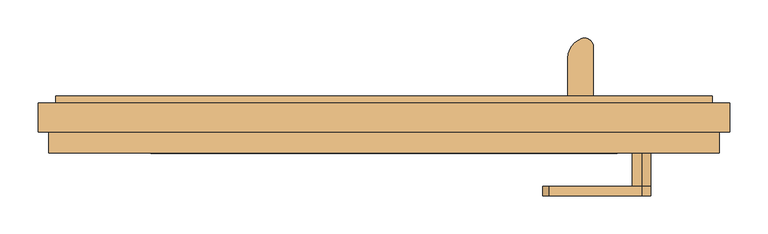
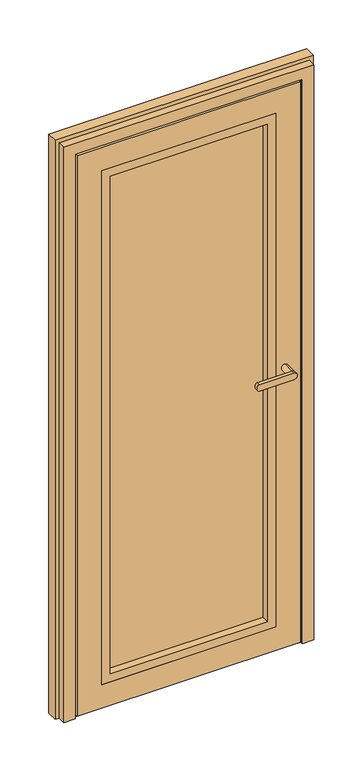
"""IFC4 building model written with IfcOpenShell, lengths in millimetres: door geometry, Schueco_FWS_ADS-75-BL-SimplySmart_inw_Family-01 : FWS SI insert unit."""

from ifc_helpers import new_model, si_unit, point, frame, frame_2d, origin, place, context, project, spatial, polyline, circle_curve, ellipse_curve, trimmed, segment, composite_curve, outline, extrude, faceted_brep, source, transform, mapped, element, save
from ifc_brep_helpers import plane_surface, cylinder_surface, extruded_surface, advanced_brep


def door_fb62e3df(model_context):
    return source(origin(), model_context, "Body", "SolidModel", [
        extrude(outline(composite_curve([segment(polyline([(241.3327032, 8.9997177), (241.3327032, 59.1618682)]), True, "CONTINUOUS"), segment(trimmed(circle_curve(frame_2d((268.5111209, 59.1618682)), 27.1784177), [point((241.3327032, 59.1618682))], [point((258.9740253, 84.6120194))], False, "CARTESIAN"), True, "CONTINUOUS"), segment(trimmed(circle_curve(frame_2d((263.0515262, 73.7310321)), 11.6198924), [point((258.9740253, 84.6120194))], [point((274.6714186, 73.7310321))], False, "CARTESIAN"), True, "CONTINUOUS"), segment(polyline([(274.6714186, 73.7310321), (274.6714186, 8.9997177), (241.3327032, 8.9997177)]), True, "CONTINUOUS")], self_intersect=False)), frame((0.0, 0.0, 2036.9340013), z_axis=(0.0, 0.0, 1.0), x_axis=(1.0, 0.0, 0.0)), (0.0, 0.0, 1.0), 4.0),
        extrude(outline(polyline([(241.3327032, 12.9997177), (274.6714186, 12.9997177), (274.6714186, 8.9997177), (241.3327032, 8.9997177), (241.3327032, 12.9997177)])), frame((0.0, 0.0, 2006.9340013), z_axis=(0.0, 0.0, 1.0), x_axis=(1.0, 0.0, 0.0)), (0.0, 0.0, 1.0), 30.0),
        extrude(outline(polyline([(241.3327032, 12.9997177), (274.6714186, 12.9997177), (274.6714186, 8.9997177), (241.3327032, 8.9997177), (241.3327032, 12.9997177)])), frame((0.0, 0.0, 56.9340013), z_axis=(0.0, 0.0, 1.0), x_axis=(1.0, 0.0, 0.0)), (0.0, 0.0, 1.0), 30.0),
        extrude(outline(composite_curve([segment(polyline([(241.3327032, 8.9997177), (241.3327032, 59.1618682)]), True, "CONTINUOUS"), segment(trimmed(circle_curve(frame_2d((268.5111209, 59.1618682)), 27.1784177), [point((241.3327032, 59.1618682))], [point((258.9740253, 84.6120194))], False, "CARTESIAN"), True, "CONTINUOUS"), segment(trimmed(circle_curve(frame_2d((263.0515262, 73.7310321)), 11.6198924), [point((258.9740253, 84.6120194))], [point((274.6714186, 73.7310321))], False, "CARTESIAN"), True, "CONTINUOUS"), segment(polyline([(274.6714186, 73.7310321), (274.6714186, 8.9997177), (241.3327032, 8.9997177)]), True, "CONTINUOUS")], self_intersect=False)), frame((0.0, 0.0, 52.9340013), z_axis=(0.0, 0.0, 1.0), x_axis=(1.0, 0.0, 0.0)), (0.0, 0.0, 1.0), 4.0),
        advanced_brep(
        [(270.7171028, 57.5977179, 2036.9340013), (245.2829507, 72.2821425, 2036.9340013), (270.7171028, 57.5977179, 56.9340013), (245.2829507, 72.2821425, 56.9340013)],
        [
            (0, 1, ellipse_curve(frame((258.0000268, 64.9399302, 2036.9340013), z_axis=(0.0, 0.0, 1.0000000000000002), x_axis=(0.5000002582658958, 0.866025254674503, 0.0)), 21.5840887, 14.6844171)),
            (1, 0, ellipse_curve(frame((258.0000268, 64.9399302, 2036.9340013), z_axis=(0.0, 0.0, 1.0000000000000002), x_axis=(0.5000002582658958, 0.866025254674503, 0.0)), 21.5840887, 14.6844171)),
            (2, 3, ellipse_curve(frame((258.0000268, 64.9399302, 56.9340013), z_axis=(0.0, 0.0, -1.0000000000000002), x_axis=(-0.866025254674503, 0.5000002582658958, 0.0)), 14.6844171, 21.5840887)),
            (3, 2, ellipse_curve(frame((258.0000268, 64.9399302, 56.9340013), z_axis=(0.0, 0.0, -1.0000000000000002), x_axis=(-0.866025254674503, 0.5000002582658958, 0.0)), 14.6844171, 21.5840887)),
            (0, 2),
            (3, 1),
        ],
        [
            plane_surface(frame((245.2829507, 72.2821425, 2036.9340013), z_axis=(0.0, 0.0, 1.0000000000000002), x_axis=(0.5000002582658958, 0.866025254674503, 0.0))),
            plane_surface(frame((245.2829507, 72.2821425, 56.9340013), z_axis=(0.0, 0.0, -1.0000000000000002), x_axis=(-0.5000002582658958, -0.866025254674503, 0.0))),
            extruded_surface(trimmed(ellipse_curve(frame((258.0000268, 64.9399302, 56.9340013), z_axis=(0.0, 0.0, -1.0000000000000002), x_axis=(-0.866025254674503, 0.5000002582658958, 0.0)), 14.6844171, 21.5840887), [point((245.2829507, 72.2821425, 56.9340013))], [point((270.7171028, 57.5977179, 56.9340013))], True, "CARTESIAN"), (0.0, 0.0, -1980.0), 1980.0),
            extruded_surface(trimmed(ellipse_curve(frame((258.0000268, 64.9399302, 56.9340013), z_axis=(0.0, 0.0, -1.0000000000000002), x_axis=(-0.866025254674503, 0.5000002582658958, 0.0)), 14.6844171, 21.5840887), [point((270.7171028, 57.5977179, 56.9340013))], [point((245.2829507, 72.2821425, 56.9340013))], True, "CARTESIAN"), (0.0, 0.0, -1980.0), 1980.0),
        ],
        [
            (0, [[1, 2]]),
            (1, [[3, 4]]),
            (2, [[5, -4, 6, -1]]),
            (3, [[-6, -3, -5, -2]]),
        ],
    ),
        advanced_brep(
        [(338.0000268, -122.0002518, 1038.0113692), (338.0000268, -122.0002518, 1061.9886308), (216.3382342, -122.0002518, 1061.9886308), (216.3382342, -122.0002518, 1038.0113692), (338.0000268, -109.5001648, 1061.9886308), (338.0000268, -109.5001648, 1038.0113692), (216.3382342, -109.5001648, 1038.0113692), (216.3382342, -109.5001648, 1061.9886308), (338.0000268, -66.0002823, 1038.0113692), (338.0000268, -66.0002823, 1061.9886308)],
        [
            (0, 1, circle_curve(frame((338.0000268, -122.0002518, 1050.0), z_axis=(0.0, -1.0, 0.0), x_axis=(0.0, 0.0, 1.0)), 11.9886308)),
            (1, 2),
            (2, 3, ellipse_curve(frame((216.3382342, -122.0002518, 1050.0), z_axis=(0.0, -1.0, 0.0), x_axis=(0.0, 0.0, -1.0)), 11.9886308, 7.9050795)),
            (3, 0),
            (4, 5, circle_curve(frame((338.0000268, -109.5001648, 1050.0), z_axis=(0.0, -1.0, 0.0), x_axis=(0.0, 0.0, 1.0)), 11.9886308)),
            (5, 6),
            (6, 7, ellipse_curve(frame((216.3382342, -109.5001648, 1050.0), z_axis=(0.0, 1.0, 0.0), x_axis=(0.0, 0.0, -1.0)), 11.9886308, 7.9050795)),
            (7, 4),
            (3, 6),
            (5, 0),
            (2, 7),
            (1, 4),
            (5, 4, circle_curve(frame((338.0000268, -109.5001648, 1050.0), z_axis=(0.0, -1.0, 0.0), x_axis=(0.0, 0.0, 1.0)), 11.9886308)),
            (8, 9, circle_curve(frame((338.0000268, -66.0002823, 1050.0), z_axis=(0.0, 1.0, 0.0), x_axis=(0.0, 0.0, 1.0)), 11.9886308)),
            (9, 8, circle_curve(frame((338.0000268, -66.0002823, 1050.0), z_axis=(0.0, 1.0, 0.0), x_axis=(0.0, 0.0, 1.0)), 11.9886308)),
            (8, 5),
            (4, 9),
        ],
        [
            plane_surface(frame((216.3382342, -122.0002518, 1038.0113692), z_axis=(0.0, -1.0, 0.0), x_axis=(-1.0, 0.0, 0.0))),
            plane_surface(frame((216.3382342, -109.5001648, 1038.0113692), z_axis=(0.0, 1.0, 0.0), x_axis=(1.0, 0.0, 0.0))),
            plane_surface(frame((338.0000268, -122.0002518, 1038.0113692), z_axis=(0.0, 0.0, -1.0), x_axis=(0.0, 1.0, 0.0))),
            extruded_surface(trimmed(ellipse_curve(frame((216.3382342, -109.5001648, 1050.0), z_axis=(0.0, 1.0, 0.0), x_axis=(0.0, 0.0, -1.0)), 11.9886308, 7.9050795), [point((216.3382342, -109.5001648, 1038.0113692))], [point((216.3382342, -109.5001648, 1061.9886308))], True, "CARTESIAN"), (0.0, 12.500086999999994, 0.0), 12.500086999999994),
            plane_surface(frame((216.3382342, -122.0002518, 1061.9886308), z_axis=(0.0, 0.0, 1.0), x_axis=(0.0, 1.0, 0.0))),
            cylinder_surface(frame((338.0000268, -109.5001648, 1050.0), z_axis=(0.0, -1.0, 0.0), x_axis=(0.0, 0.0, 1.0)), 11.9886308),
            plane_surface(frame((338.0000268, -66.0002823, 1061.9886308), z_axis=(0.0, 1.0, 0.0), x_axis=(-1.0, 0.0, 0.0))),
            cylinder_surface(frame((338.0000268, -66.0002823, 1050.0), z_axis=(0.0, -1.0, 0.0), x_axis=(0.0, 0.0, 1.0)), 11.9886308),
        ],
        [
            (0, [[1, 2, 3, 4]]),
            (1, [[5, 6, 7, 8]]),
            (2, [[9, -6, 10, -4]]),
            (3, [[11, -7, -9, -3]]),
            (4, [[12, -8, -11, -2]]),
            (5, [[-10, 13, -12, -1]]),
            (6, [[14, 15]]),
            (7, [[16, -5, 17, -14]]),
            (7, [[-17, -13, -16, -15]]),
        ],
    ),
        extrude(outline(polyline([(95.0, 306.0000268), (2006.0, 306.0000268), (2006.0, -305.9999732), (95.0, -305.9999732), (95.0, 306.0000268)]), holes=[polyline([(125.0, -275.9999732), (1976.0, -275.9999732), (1976.0, 276.0000268), (125.0, 276.0000268), (125.0, -275.9999732)])]), frame((0.0, -66.0002823, 0.0), z_axis=(0.0, 1.0, 0.0), x_axis=(0.0, 0.0, 1.0)), (0.0, 0.0, 1.0), 26.0000097),
        faceted_brep([(-392.9999732, -66.0002823, 2093.0), (-392.9999732, -57.5000065, 2093.0), (-392.9999732, -57.5000065, 8.0), (-392.9999732, -66.0002823, 8.0), (393.0000268, -57.5000065, 8.0), (393.0000268, -66.0002823, 8.0), (393.0000268, -57.5000065, 2093.0), (371.0000268, -57.5000065, 30.0), (371.0000268, -57.5000065, 2071.0), (-370.9999732, -57.5000065, 2071.0), (-370.9999732, -57.5000065, 30.0), (393.0000268, -66.0002823, 2093.0), (-305.9999732, -66.0002823, 95.0), (-305.9999732, -66.0002823, 2006.0), (306.0000268, -66.0002823, 2006.0), (306.0000268, -66.0002823, 95.0), (-305.9999732, -2.0002726, 2006.0), (-305.9999732, -2.0002726, 95.0), (306.0000268, -2.0002726, 95.0), (306.0000268, -2.0002726, 2006.0), (-273.9999732, -2.0002726, 127.0), (-273.9999732, -2.0002726, 1974.0), (274.0000268, -2.0002726, 1974.0), (274.0000268, -2.0002726, 127.0), (-273.9999732, 8.9997177, 1974.0), (-273.9999732, 8.9997177, 127.0), (274.0000268, 8.9997177, 127.0), (274.0000268, 8.9997177, 1974.0), (-360.9999732, 8.9997177, 40.0), (-360.9999732, 8.9997177, 2061.0), (361.0000268, 8.9997177, 2061.0), (361.0000268, 8.9997177, 40.0), (-360.9999732, 0.4997603, 2061.0), (-360.9999732, 0.4997603, 40.0), (361.0000268, 0.4997603, 40.0), (361.0000268, 0.4997603, 2061.0), (-370.9999732, 0.4997603, 30.0), (-370.9999732, 0.4997603, 2071.0), (371.0000268, 0.4997603, 2071.0), (371.0000268, 0.4997603, 30.0)], [[[0, 1, 2, 3]], [[3, 2, 4, 5]], [[2, 1, 6, 4], [7, 8, 9, 10]], [[5, 4, 6, 11]], [[5, 11, 0, 3], [12, 13, 14, 15]], [[16, 13, 12, 17]], [[17, 12, 15, 18]], [[18, 15, 14, 19]], [[18, 19, 16, 17], [20, 21, 22, 23]], [[24, 21, 20, 25]], [[25, 20, 23, 26]], [[26, 23, 22, 27]], [[28, 29, 30, 31], [26, 27, 24, 25]], [[32, 29, 28, 33]], [[33, 28, 31, 34]], [[34, 31, 30, 35]], [[36, 37, 38, 39], [34, 35, 32, 33]], [[9, 37, 36, 10]], [[10, 36, 39, 7]], [[7, 39, 38, 8]], [[11, 6, 1, 0]], [[19, 14, 13, 16]], [[27, 22, 21, 24]], [[35, 30, 29, 32]], [[8, 38, 37, 9]]]),
        extrude(outline(polyline([(306.0000268, -40.0002726), (-305.9999732, -40.0002726), (-305.9999732, -2.0002726), (306.0000268, -2.0002726), (306.0000268, -40.0002726)])), frame((0.0, 0.0, 95.0), z_axis=(0.0, 0.0, 1.0), x_axis=(1.0, 0.0, 0.0)), (0.0, 0.0, 1.0), 1911.0),
        extrude(outline(composite_curve([segment(polyline([(-39.1486683, 30.0), (-17.8439358, 30.0), (-17.8439358, 4.0204884)]), True, "CONTINUOUS"), segment(trimmed(circle_curve(frame_2d((-28.496302, 16.1220754)), 16.1220754), [point((-17.8439358, 4.0204884))], [point((-39.1486683, 4.0204884))], False, "CARTESIAN"), True, "CONTINUOUS"), segment(polyline([(-39.1486683, 4.0204884), (-39.1486683, 30.0)]), True, "CONTINUOUS")], self_intersect=False)), frame((-370.9999732, 0.0, 0.0), z_axis=(1.0, 0.0, 0.0), x_axis=(0.0, 1.0, 0.0)), (0.0, 0.0, 1.0), 742.0),
        extrude(outline(polyline([(-360.9999732, 0.4997603), (-360.9999732, 8.9997177), (361.0000268, 8.9997177), (361.0000268, 0.4997603), (-360.9999732, 0.4997603)])), frame((0.0, 0.0, 8.0), z_axis=(0.0, 0.0, 1.0), x_axis=(1.0, 0.0, 0.0)), (0.0, 0.0, 1.0), 32.0),
        faceted_brep([(430.999943, 8.9997177, 2130.999943), (430.999943, 0.0, 2130.999943), (430.999943, 0.0, 0.0), (430.999943, 8.9997177, 0.0), (-454.0, 0.0, 0.0), (-454.0, 0.0, 2154.0), (454.0, 0.0, 2154.0), (454.0, 0.0, 0.0), (-430.999943, 0.0, 2130.999943), (-430.999943, 0.0, 0.0), (454.0, -38.0, 0.0), (440.0, -38.0, 0.0), (440.0, -66.0002823, 0.0), (399.9999732, -66.0002823, 0.0), (399.9999732, -57.5000065, 0.0), (388.4999732, -57.5000065, 0.0), (388.4999732, 0.4997603, 0.0), (367.9999732, 0.4997603, 0.0), (367.9999732, 8.9997177, 0.0), (-367.9999732, 8.9997177, 0.0), (-430.999943, 8.9997177, 0.0), (-430.999943, 8.9997177, 2130.999943), (367.9999732, 8.9997177, 2067.9999732), (-367.9999732, 8.9997177, 2067.9999732), (399.9999732, -66.0002823, 2099.9999732), (399.9999732, -57.5000065, 2099.9999732), (-399.9999732, -57.5000065, 0.0), (-388.4999732, -57.5000065, 0.0), (-388.4999732, -57.5000065, 2088.4999732), (388.4999732, -57.5000065, 2088.4999732), (-399.9999732, -57.5000065, 2099.9999732), (-440.0, -66.0002823, 0.0), (-399.9999732, -66.0002823, 0.0), (-399.9999732, -66.0002823, 2099.9999732), (440.0, -66.0002823, 2140.0), (-440.0, -66.0002823, 2140.0), (440.0, -38.0, 2140.0), (-454.0, -38.0, 0.0), (-440.0, -38.0, 0.0), (-440.0, -38.0, 2140.0), (454.0, -38.0, 2154.0), (-454.0, -38.0, 2154.0), (-367.9999732, 0.4997603, 0.0), (-388.4999732, 0.4997603, 0.0), (367.9999732, 0.4997603, 2067.9999732), (-367.9999732, 0.4997603, 2067.9999732), (388.4999732, 0.4997603, 2088.4999732), (-388.4999732, 0.4997603, 2088.4999732)], [[[0, 1, 2, 3]], [[4, 5, 6, 7, 2, 1, 8, 9]], [[3, 2, 7, 10, 11, 12, 13, 14, 15, 16, 17, 18]], [[19, 20, 21, 0, 3, 18, 22, 23]], [[24, 25, 14, 13]], [[26, 27, 28, 29, 15, 14, 25, 30]], [[31, 32, 33, 24, 13, 12, 34, 35]], [[34, 12, 11, 36]], [[37, 38, 39, 36, 11, 10, 40, 41]], [[4, 9, 20, 19, 42, 43, 27, 26, 32, 31, 38, 37]], [[20, 9, 8, 21]], [[18, 17, 44, 22]], [[42, 19, 23, 45]], [[32, 26, 30, 33]], [[31, 35, 39, 38]], [[4, 37, 41, 5]], [[6, 40, 10, 7]], [[43, 42, 45, 44, 17, 16, 46, 47]], [[16, 15, 29, 46]], [[27, 43, 47, 28]], [[21, 8, 1, 0]], [[33, 30, 25, 24]], [[35, 34, 36, 39]], [[23, 22, 44, 45]], [[5, 41, 40, 6]], [[47, 46, 29, 28]]]),
    ])


if __name__ == "__main__":
    model = new_model("IFC4")
    model_context = context("Model", 3, world=origin())
    ifc_project = project(units=[si_unit("LENGTHUNIT", "METRE", prefix="MILLI")], contexts=[model_context])
    site = spatial("IfcSite", under=ifc_project)
    building = spatial("IfcBuilding", under=site)
    placement = place(None, origin())
    door_shape = door_fb62e3df(model_context)
    element("IfcDoor", 1, ObjectType="Schueco_FWS_ADS-75-BL-SimplySmart_inw_Family-01 : FWS SI insert unit", at=placement, inside=building, context=model_context, shape_type="MappedRepresentation", body=[
        mapped(door_shape, transform((0.0, 0.0, 0.0), x_axis=(1.0, 0.0, 0.0), y_axis=(0.0, 1.0, 0.0), z_axis=(0.0, 0.0, 1.0))),
    ])
    save(model, "model.ifc")

# Revit data of these elements
# Type "Schueco_FWS_ADS-75-BL-SimplySmart_inw_Family-01 : FWS SI insert unit"
#   Type Mark = "27"
#   __NOTE__ = "Data describes the optimum values of the entire system. The properites of a selected design option have to be determined on an individual basis!"
#   Wind load resistance = "Class C3"
#   Watertightness = "Class E750"
#   Thermal insulation = "Uf = 1.6 W/(m²K)"
#   Sound insulation = "..."
#   Schueco thermal insulation standard = "Highly thermally insulated"
#   Opening type = "Inward-opening, Flush-fitted"
#   Model = "Schueco ADS 75 BL SimplySmart"
#   Mechanical loading = "..."
#   Maximum leaf width in mm = "1400"
#   Maximum leaf weight in kg = "200"
#   Maximum leaf height in mm = "3000"
#   Material = "Aluminium"
#   Construction Type = "Door, single-leaf, inward-opening"
#   Manufacturer = "Schueco International KG"
#   Long term functionality = "..."
#   Glazing data = "Triple glazing 38mm"
#   Façade insert unit = "yes"
#   Family creation date = "08.2017"
#   Description = "Schueco Aluminium Door System (ADS)"
#   Burglar resistance = "Class RC 2"
#   Areas of use = "Public buildings, Residential buildings, Side entrance"
#   Analytic Construction = "<None>"
#   Air permeability = "Class 4"
#   Width [instance default] = 1393.741 mm
#   Leaf opening angle [instance default] = 0.00°
#   IOf_T = 38 mm
#   Height [instance default] = 2280 mm
#   Glazing area [instance default] = 2.03957 m²
#   Distance from bottom to handles [instance default] = 1050 mm
#   Clear opening width [instance default] = 1221.741 mm
#   Standard threshold = no
#   Low level threshold = yes
#   Handles = yes
#   FWS SI insert unit = yes
#   FWS HI insert unit = no
#   Glass = none
#   Frame = Alu
#   Fittings = none
# Element 1 (IfcDoor, "Schueco_FWS_ADS-75-BL-SimplySmart_inw_Family-01 : FWS SI insert unit")
#   Width = 908 mm
#   Height = 2154 mm
#   Glazing area = 1.01216 m²
#   Clear opening width = 736 mm
#   Materials on its faces: "Alu", "Glass"
# Materials
#   "Alu": class "Glas", colour RGB 140 140 140, transparency 0
#   "Glass": class "Glass", colour RGB 128 128 255, transparency 0.75, Description = "Soda Lime Glass", Cost = 0
